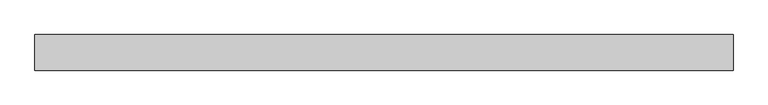
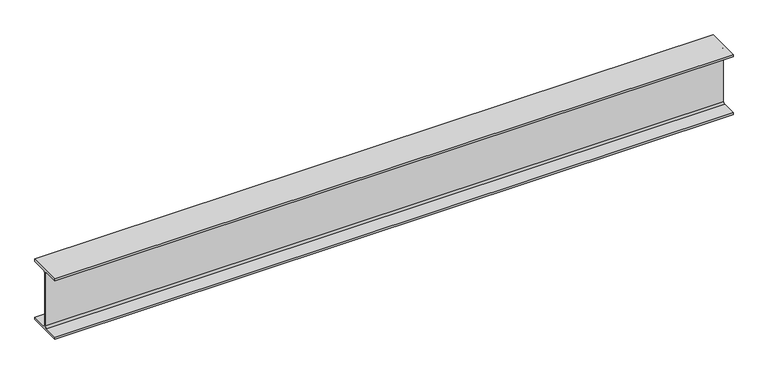
"""IFC4 building model written with IfcOpenShell, lengths in millimetres: beam geometry, Old_Steel Beam_H-KSD3502 : H_SB_ASB_H-200×200x8x12."""

from ifc_helpers import new_model, si_unit, point, frame, frame_2d, origin, place, context, project, spatial, polyline, circle_curve, trimmed, segment, composite_curve, outline, extrude, source, transform, mapped, element, save


def beam_e6466eaf(model_context):
    return source(origin(), model_context, "Body", "SweptSolid", [
        extrude(outline(composite_curve([segment(polyline([(82.5, -141.5), (82.5, -151.7), (-82.5, -151.7), (-82.5, -141.5), (-11.9, -141.5)]), True, "CONTINUOUS"), segment(trimmed(circle_curve(frame_2d((-11.9, -132.6)), 8.9), [point((-11.9, -141.5))], [point((-3.0, -132.6))], True, "CARTESIAN"), True, "CONTINUOUS"), segment(polyline([(-3.0, -132.6), (-3.0, 132.6)]), True, "CONTINUOUS"), segment(trimmed(circle_curve(frame_2d((-11.9, 132.6)), 8.9), [point((-3.0, 132.6))], [point((-11.9, 141.5))], True, "CARTESIAN"), True, "CONTINUOUS"), segment(polyline([(-11.9, 141.5), (-82.5, 141.5), (-82.5, 151.7), (82.5, 151.7), (82.5, 141.5), (11.9, 141.5)]), True, "CONTINUOUS"), segment(trimmed(circle_curve(frame_2d((11.9, 132.6)), 8.9), [point((11.9, 141.5))], [point((3.0, 132.6))], True, "CARTESIAN"), True, "CONTINUOUS"), segment(polyline([(3.0, 132.6), (3.0, -132.6)]), True, "CONTINUOUS"), segment(trimmed(circle_curve(frame_2d((11.9, -132.6)), 8.9), [point((3.0, -132.6))], [point((11.9, -141.5))], True, "CARTESIAN"), True, "CONTINUOUS"), segment(polyline([(11.9, -141.5), (82.5, -141.5)]), True, "CONTINUOUS")], self_intersect=False)), frame((-1409.9859537, 0.0, 0.0), z_axis=(1.0, 0.0, 0.0), x_axis=(0.0, 1.0, 0.0)), (0.0, 0.0, 1.0), 3231.4633723),
    ])


if __name__ == "__main__":
    model = new_model("IFC4")
    model_context = context("Model", 3, world=origin())
    ifc_project = project(units=[si_unit("LENGTHUNIT", "METRE", prefix="MILLI")], contexts=[model_context])
    site = spatial("IfcSite", under=ifc_project)
    building = spatial("IfcBuilding", under=site)
    placement = place(None, origin())
    beam_shape = beam_e6466eaf(model_context)
    element("IfcBeam", 1, ObjectType="Old_Steel Beam_H-KSD3502 : H_SB_ASB_H-200×200x8x12", at=placement, inside=building, context=model_context, shape_type="MappedRepresentation", body=[
        mapped(beam_shape, transform((0.0, 0.0, 0.0), x_axis=(1.0, 0.0, 0.0), y_axis=(0.0, 1.0, 0.0), z_axis=(0.0, 0.0, 1.0))),
    ])
    save(model, "model.ifc")

# Revit data of these elements
# Type "Old_Steel Beam_H-KSD3502 : H_SB_ASB_H-200×200x8x12"
#   Width = 20.0 cm
#   Web Thickness = 0.8 cm
#   Web Fillet = 1.3 cm
#   Warping Constant = 141376.0 cm⁶
#   Torsional Moment of Inertia = 26.2485 cm⁴
#   Torsional Modulus = 1.0 cm³
#   Section Area = 63.53 cm²
#   Plastic Modulus weak axis = 244.0 cm³
#   Plastic Modulus strong axis = 525.0 cm³
#   Perimeter = 1.16 m²/m
#   Nominal Weight = 49.90 kgf/m
#   Moment of Inertia weak axis = 1600.00 cm⁴
#   Moment of Inertia strong axis = 4720.00 cm⁴
#   Height = 20.0 cm
#   Flange Thickness = 1.2 cm
#   Elastic Modulus weak axis = 160.0 cm³
#   Elastic Modulus strong axis = 472.0 cm³
#   Centroid Vertical = 10.0 cm
#   Centroid Horizontal = 10.0 cm
#   Length [instance default] = 1.5240 m
#   Structural Material [instance default] = Steel, 45-345
#   Assembly Code = ""
# Element 1 (IfcBeam, "Old_Steel Beam_H-KSD3502 : H_SB_ASB_H-200×200x8x12")
#   Structural Material = none
# Materials
#   "Steel, 45-345": class "Metal", colour RGB 189 187 185, transparency 0, Description = "Steel 345 MPa", Cost = 0
